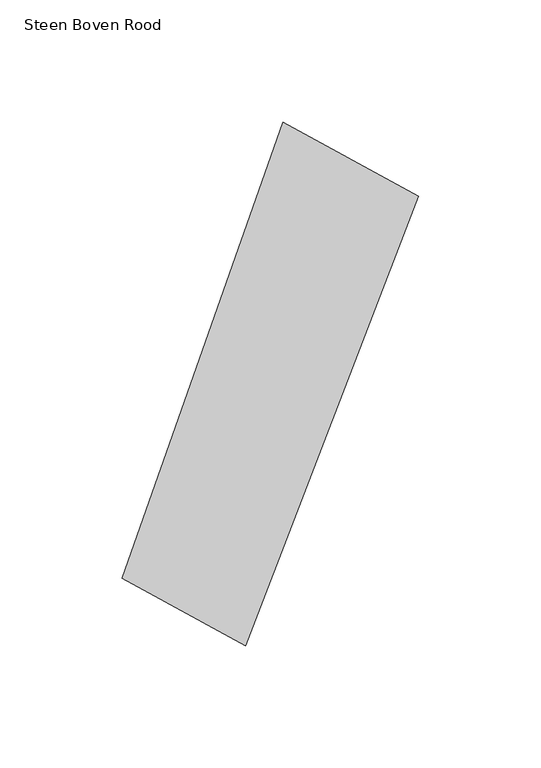
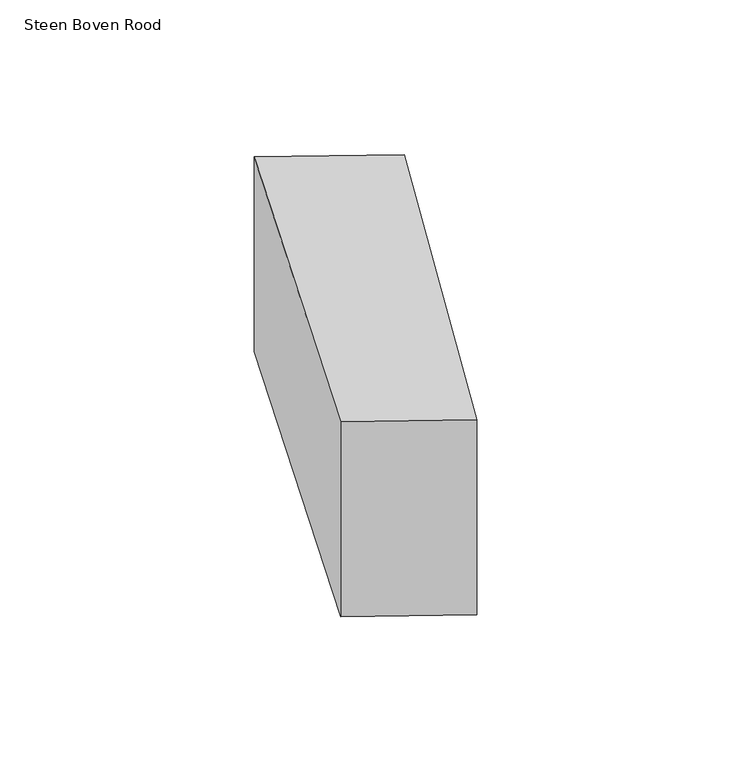
"""IFC4 building model written with IfcOpenShell, lengths in millimetres: proxy geometry, 00_GMA_steen_versie_4 : Steen Boven Rood."""

from ifc_helpers import new_model, si_unit, origin, origin_with_axes, place, context, project, spatial, polyline, outline, extrude, source, transform, mapped, element, save


def steen_boven_rood_6278fd23(model_context):
    return source(origin(), model_context, "Body", "SweptSolid", [
        extrude(outline(polyline([(137.4465391, 165.0969337), (66.67604, -18.4568784), (16.2851371, 8.9720056), (82.0544979, 195.2701005), (137.4465391, 165.0969337)])), origin_with_axes(), (0.0, 0.0, 1.0), 100.0),
    ])


if __name__ == "__main__":
    model = new_model("IFC4")
    model_context = context("Model", 3, world=origin())
    ifc_project = project(units=[si_unit("LENGTHUNIT", "METRE", prefix="MILLI")], contexts=[model_context])
    site = spatial("IfcSite", under=ifc_project)
    building = spatial("IfcBuilding", under=site)
    placement = place(None, origin())
    steen_boven_rood_shape = steen_boven_rood_6278fd23(model_context)
    element("IfcBuildingElementProxy", 1, Name="00_GMA_steen_versie_4 : Steen Boven Rood", ObjectType="00_GMA_steen_versie_4 : Steen Boven Rood", at=placement, inside=building, context=model_context, shape_type="MappedRepresentation", body=[
        mapped(steen_boven_rood_shape, transform((0.0, 0.0, 0.0), x_axis=(1.0, 0.0, 0.0), y_axis=(0.0, 1.0, 0.0), z_axis=(0.0, 0.0, 1.0))),
    ])
    save(model, "model.ifc")

# Revit data of these elements
# Type "00_GMA_steen_versie_4 : Steen Boven Rood"
#   StootVoegHalfBoven [instance default] = 5 mm
#   StootVoegHalf [instance default] = 5 mm
#   StootVoegBreedteOnder = 10 mm
#   StootVoegBreedteBoven = 10 mm
#   Steendikte = 100 mm
#   LintVoegOnderHalf = 5 mm
#   LintVoegOnder = 10 mm
#   LintVoegBovenHalf = 0 mm
#   LintVoegBoven = 0 mm
#   materiaal = 21_steen_rood
#   MateriaalVoeg = none
#   Default Elevation = 0
# Element 1 (IfcBuildingElementProxy, "00_GMA_steen_versie_4 : Steen Boven Rood")
#   Materials on its faces: "21_steen_rood"
# Materials
#   "21_steen_rood": class "Unassigned", colour RGB 213 111 43, transparency 0, Cost = 0
